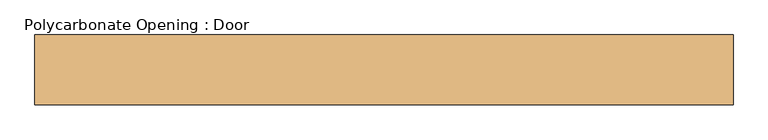
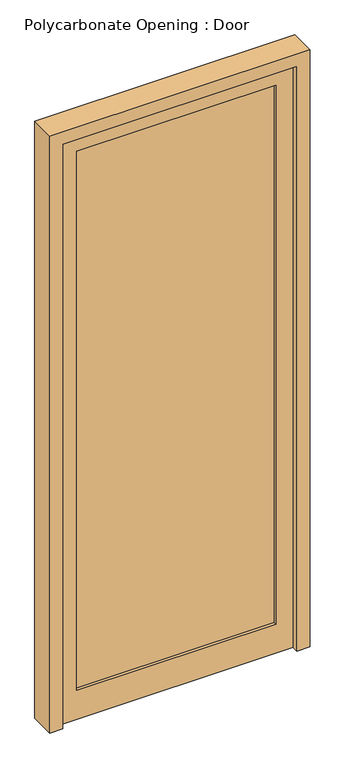
"""IFC4 building model written with IfcOpenShell, lengths in millimetres: door geometry, Polycarbonate Opening : Door."""

from ifc_helpers import new_model, si_unit, frame, origin, place, context, project, spatial, polyline, outline, extrude, source, transform, mapped, element, save


def polycarbonate_opening_door_ee853a28(model_context):
    return source(origin(), model_context, "Body", "SweptSolid", [
        extrude(outline(polyline([(457.2, 0.0), (-457.2, 0.0), (-457.2, 25.4), (457.2, 25.4), (457.2, 0.0)])), frame((0.0, 0.0, 50.8), z_axis=(0.0, 0.0, 1.0), x_axis=(1.0, 0.0, 0.0)), (0.0, 0.0, 1.0), 2360.0132885),
        extrude(outline(polyline([(2410.8132885, -457.2), (0.0, -457.2), (0.0, 457.2), (2410.8132885, 457.2), (2410.8132885, -457.2)]), holes=[polyline([(119.0625, 388.9375), (119.0625, -388.9375), (2342.5507885, -388.9375), (2342.5507885, 388.9375), (119.0625, 388.9375)])]), frame((0.0, -12.7, 0.0), z_axis=(0.0, 1.0, 0.0), x_axis=(0.0, 0.0, 1.0)), (0.0, 0.0, 1.0), 50.8),
        extrude(outline(polyline([(2461.6132885, 508.0), (2461.6132885, -508.0), (0.0, -508.0), (0.0, -457.2), (2410.8132885, -457.2), (2410.8132885, 457.2), (0.0, 457.2), (0.0, 508.0), (2461.6132885, 508.0)])), frame((0.0, -38.1, 0.0), z_axis=(0.0, 1.0, 0.0), x_axis=(0.0, 0.0, 1.0)), (0.0, 0.0, 1.0), 101.6),
    ])


if __name__ == "__main__":
    model = new_model("IFC4")
    model_context = context("Model", 3, world=origin())
    ifc_project = project(units=[si_unit("LENGTHUNIT", "METRE", prefix="MILLI")], contexts=[model_context])
    site = spatial("IfcSite", under=ifc_project)
    building = spatial("IfcBuilding", under=site)
    placement = place(None, origin())
    polycarbonate_opening_door_shape = polycarbonate_opening_door_ee853a28(model_context)
    element("IfcDoor", 1, ObjectType="Polycarbonate Opening : Door", at=placement, inside=building, context=model_context, shape_type="MappedRepresentation", body=[
        mapped(polycarbonate_opening_door_shape, transform((0.0, 0.0, 0.0), x_axis=(1.0, 0.0, 0.0), y_axis=(0.0, 1.0, 0.0), z_axis=(0.0, 0.0, 1.0))),
    ])
    save(model, "model.ifc")

# Revit data of these elements
# Type "Polycarbonate Opening : Door"
#   Type Mark = "60"
#   OD_DS_Door_Material = "ALUM./GLAZING"
#   OD_DS_Door_Type = "STOREFRONT (NARROW STILE)"
#   OD_DS_Lockset = "ENTRY LOCK (INSIDE ADA LEVER ALWAYS ACTIVE)"
#   Analytic Construction = "<None>"
#   offset [instance default] = 0' - 0 1/2"
#   Stile = 0' - 2 11/16"
#   Mullion Width = 0' - 2"
#   Mullion Depth = 0' - 4"
#   Opening Size [instance default] = 5' - 1.50212"
#   Door Width [instance default] = 5' - 1.50212"
#   Window ON/OFF = yes
#   Door On/Off = no
#   Mullion Material = KAWNEER 260 INSULCLADTM THERMAL ENTRANCE - CLEAR ANODIZED ALUM.
#   Glass Material = TEMPERED INSULATED GLAZING (CARDINAL GLASS LoĒ²-240\nOR EQUIVALENT)
#   Door Material = KAWNEER 260 INSULCLADTM THERMAL ENTRANCE - CLEAR ANODIZED ALUM.
# Element 1 (IfcDoor, "Polycarbonate Opening : Door")
#   Materials on its faces: "KAWNEER 260 INSULCLADTM THERMAL ENTRANCE - CLEAR ANODIZED ALUM.", "TEMPERED INSULATED GLAZING (CARDINAL GLASS LoĒ²-240\nOR EQUIVALENT)"
# Materials
#   "KAWNEER 260 INSULCLADTM THERMAL ENTRANCE - CLEAR ANODIZED ALUM.": class "Metal", colour RGB 244 244 244, transparency 0, Description = "Aluminum 6061", Cost = 0
#   "TEMPERED INSULATED GLAZING (CARDINAL GLASS LoĒ²-240\nOR EQUIVALENT)": class "Glass", colour RGB 196 205 210, transparency 0.85, Description = "Soda Lime Glass", Cost = 0
